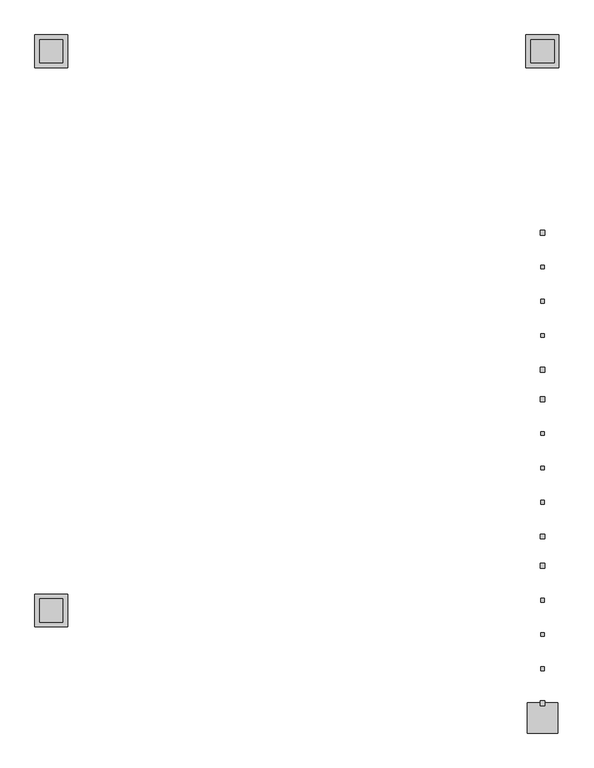
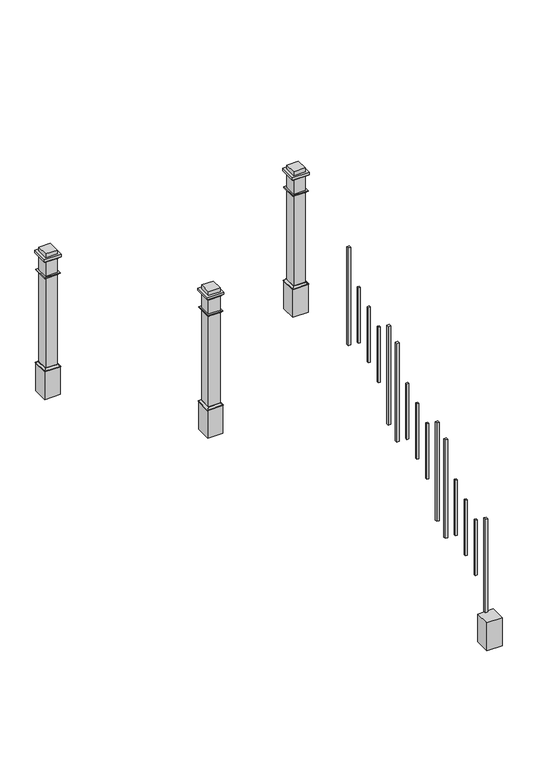
"""IFC4 building model written with IfcOpenShell, lengths in millimetres: railing geometry."""

import ifcopenshell
import ifcopenshell.guid

model = None  # the IFC model being written
_history = None  # IfcOwnerHistory: only IFC2X3 demands one
_inside = {}  # id of a spatial element -> (the spatial element, [elements in it])
_under = {}  # id of a project, library or spatial element -> (it, [spatial elements below it])
_declared = {}  # id of a project -> (the project, [libraries it declares])
_typed = {}  # id of a type object -> (the type object, [elements of that type])
_made_of = {}  # id of a material, layer set ... -> (it, [elements and type objects made of it])


def new_model(schema):
    """Start an empty IFC model of exactly this schema.

    Asked for "IFC4X3", IfcOpenShell would pick the latest addendum, in which some entities
    have other attributes; the version numbers below select the first issue.
    IFC2X3 requires an IfcOwnerHistory on every rooted entity: one is made here for all.
    """
    global model, _history
    if schema == "IFC4X3":
        model = ifcopenshell.file(schema_version=(4, 3, 0, 0))
    else:
        model = ifcopenshell.file(schema=schema)
    _inside.clear()
    _under.clear()
    _declared.clear()
    _typed.clear()
    _made_of.clear()
    _history = None
    if model.schema == "IFC2X3":
        org = make("IfcOrganization", Name="unknown")
        user = make(
            "IfcPersonAndOrganization",
            ThePerson=make("IfcPerson", FamilyName="unknown"),
            TheOrganization=org,
        )
        app = make(
            "IfcApplication",
            ApplicationDeveloper=org,
            Version="unknown",
            ApplicationFullName="unknown",
            ApplicationIdentifier="unknown",
        )
        _history = make(
            "IfcOwnerHistory",
            OwningUser=user,
            OwningApplication=app,
            ChangeAction="ADDED",
            CreationDate=0,
        )
    return model


def make(cls, **values):
    """One entity of the class cls with the attributes given. An attribute that is None is left unset."""
    return model.create_entity(
        cls, **{name: value for name, value in values.items() if value is not None}
    )


def rooted(cls, **values):
    """An entity with a GlobalId (a new one), such as an element, a storey or a relation."""
    return make(cls, GlobalId=ifcopenshell.guid.new(), OwnerHistory=_history, **values)


def si_unit(unit_type, name, prefix=None):
    """IfcSIUnit, for example si_unit("LENGTHUNIT", "METRE", prefix="MILLI")."""
    return make("IfcSIUnit", UnitType=unit_type, Prefix=prefix, Name=name)


def assignment(units):
    """IfcUnitAssignment: the units of a project."""
    return None if units is None else make("IfcUnitAssignment", Units=units)


def point(xyz):
    """IfcCartesianPoint."""
    return None if xyz is None else make("IfcCartesianPoint", Coordinates=xyz)


def direction(xyz):
    """IfcDirection."""
    return None if xyz is None else make("IfcDirection", DirectionRatios=xyz)


def frame(location, z_axis=None, x_axis=None):
    """IfcAxis2Placement3D, a coordinate frame: its origin and axes. An axis left out is left unset."""
    return make(
        "IfcAxis2Placement3D",
        Location=point(location),
        Axis=direction(z_axis),
        RefDirection=direction(x_axis),
    )


def origin():
    """The frame at (0, 0, 0) with its axes left unset."""
    return frame((0.0, 0.0, 0.0))


def place(relative_to, where):
    """IfcLocalPlacement: puts the frame where relative to a parent placement (None: the world)."""
    return make(
        "IfcLocalPlacement", PlacementRelTo=relative_to, RelativePlacement=where
    )


def context(
    kind, dimensions, precision=None, world=None, true_north=None, identifier=None
):
    """IfcGeometricRepresentationContext, for example the 3D "Model" context."""
    return make(
        "IfcGeometricRepresentationContext",
        ContextIdentifier=identifier,
        ContextType=kind,
        CoordinateSpaceDimension=dimensions,
        Precision=precision,
        WorldCoordinateSystem=world,
        TrueNorth=true_north,
    )


def project(units=None, contexts=None):
    """IfcProject with its units and contexts."""
    return rooted(
        "IfcProject",
        Name="project",
        RepresentationContexts=contexts,
        UnitsInContext=assignment(units),
    )


def spatial(cls, under=None, at=None, **own):
    """A site, building, storey or space (cls), placed at a placement, below another one or the project."""
    s = rooted(cls, ObjectPlacement=at, **own)
    if under is not None:
        _under.setdefault(under.id(), (under, []))[1].append(s)
    return s


def polyline(points):
    """IfcPolyline through the points."""
    return make("IfcPolyline", Points=[point(p) for p in points])


def ellipse_curve(where, semi_axis1, semi_axis2):
    """IfcEllipse in the frame where."""
    return make(
        "IfcEllipse", Position=where, SemiAxis1=semi_axis1, SemiAxis2=semi_axis2
    )


def outline(outer, holes=None, kind="AREA"):
    """IfcArbitraryClosedProfileDef: a profile drawn as a closed curve; with holes, ...WithVoids."""
    if holes is None:
        return make("IfcArbitraryClosedProfileDef", ProfileType=kind, OuterCurve=outer)
    return make(
        "IfcArbitraryProfileDefWithVoids",
        ProfileType=kind,
        OuterCurve=outer,
        InnerCurves=holes,
    )


def extrude(swept, where, along, depth):
    """IfcExtrudedAreaSolid: the profile swept, set in the frame where, extruded along a direction by depth."""
    return make(
        "IfcExtrudedAreaSolid",
        SweptArea=swept,
        Position=where,
        ExtrudedDirection=direction(along),
        Depth=depth,
    )


def faces_of(points, faces, orient=None, outer=None):
    """IfcFace entities. A face is a list of loops; a loop is a list of indices into points, from 0.

    orient and outer hold one flag for each loop. By default every Orientation is true, the
    first loop of a face is its IfcFaceOuterBound and the others are IfcFaceBound.
    """
    made = []
    for i, loops in enumerate(faces):
        bounds = []
        for j, loop in enumerate(loops):
            is_outer = j == 0 if outer is None else outer[i][j]
            bounds.append(
                make(
                    "IfcFaceOuterBound" if is_outer else "IfcFaceBound",
                    Bound=make("IfcPolyLoop", Polygon=[points[k] for k in loop]),
                    Orientation=True if orient is None else orient[i][j],
                )
            )
        made.append(make("IfcFace", Bounds=bounds))
    return made


def faceted_brep(points, faces, orient=None, outer=None, voids=None):
    """IfcFacetedBrep: a solid bounded by flat faces; with voids (closed shells), ...WithVoids."""
    shared = [point(p) for p in points]
    hull = make("IfcClosedShell", CfsFaces=faces_of(shared, faces, orient, outer))
    if voids is None:
        return make("IfcFacetedBrep", Outer=hull)
    return make(
        "IfcFacetedBrepWithVoids",
        Outer=hull,
        Voids=[
            make(cls, CfsFaces=faces_of(shared, fs, o, b)) for cls, fs, o, b in voids
        ],
    )


def shape(context_of_items, identifier, shape_type, items):
    """IfcShapeRepresentation: the items that make up one representation, for example the "Body"."""
    return make(
        "IfcShapeRepresentation",
        ContextOfItems=context_of_items,
        RepresentationIdentifier=identifier,
        RepresentationType=shape_type,
        Items=items,
    )


def source(mapping_origin, context_of_items, identifier, shape_type, items):
    """IfcRepresentationMap: a shape defined once, which mapped items show again and again."""
    return make(
        "IfcRepresentationMap",
        MappingOrigin=mapping_origin,
        MappedRepresentation=shape(context_of_items, identifier, shape_type, items),
    )


def transform(
    local_origin,
    x_axis=None,
    y_axis=None,
    z_axis=None,
    scale=None,
    scale2=None,
    scale3=None,
    uniform=True,
):
    """IfcCartesianTransformationOperator3D, or its non-uniform kind. x_axis, y_axis, z_axis: its Axis1, 2, 3."""
    if uniform:
        return make(
            "IfcCartesianTransformationOperator3D",
            Axis1=direction(x_axis),
            Axis2=direction(y_axis),
            LocalOrigin=point(local_origin),
            Scale=scale,
            Axis3=direction(z_axis),
        )
    return make(
        "IfcCartesianTransformationOperator3DnonUniform",
        Axis1=direction(x_axis),
        Axis2=direction(y_axis),
        LocalOrigin=point(local_origin),
        Scale=scale,
        Axis3=direction(z_axis),
        Scale2=scale2,
        Scale3=scale3,
    )


def mapped(mapping_source, mapping_target):
    """IfcMappedItem: shows the shape of a source again, moved by a transform."""
    return make(
        "IfcMappedItem", MappingSource=mapping_source, MappingTarget=mapping_target
    )


def made_of(thing, what):
    """Note that an element or type object is made of a material, layer set ...; save() writes the relation."""
    if what is not None:
        _made_of.setdefault(what.id(), (what, []))[1].append(thing)
    return thing


def element(
    cls,
    number,
    at=None,
    inside=None,
    cuts=None,
    type_object=None,
    material=None,
    context=None,
    identifier="Body",
    shape_type=None,
    held_by="IfcProductDefinitionShape",
    body=None,
    shapes=None,
    **own,
):
    """One element of the class cls, such as IfcWall. Its Tag is "e" and its number.

    at: its placement. inside: the storey or other place that contains it. cuts: it is an
    opening in that element (IfcRelVoidsElement). A single representation is given by context,
    identifier, shape_type and body (its items); several are given by shapes. held_by: the class
    of the entity that holds the representations. save() writes the other relations.
    """
    e = rooted(cls, Tag="e%d" % number, ObjectPlacement=at, **own)
    if body is not None:
        shapes = [shape(context, identifier, shape_type, body)]
    if shapes is not None:
        e.Representation = make(held_by, Representations=shapes)
    if inside is not None:
        _inside.setdefault(inside.id(), (inside, []))[1].append(e)
    if cuts is not None:
        rooted(
            "IfcRelVoidsElement", RelatingBuildingElement=cuts, RelatedOpeningElement=e
        )
    if type_object is not None:
        _typed.setdefault(type_object.id(), (type_object, []))[1].append(e)
    return made_of(e, material)


def aggregate(whole, parts):
    """IfcRelAggregates: a whole, such as a stair, and the parts it consists of."""
    return rooted("IfcRelAggregates", RelatingObject=whole, RelatedObjects=parts)


def save(model, path):
    """Write the relations noted so far, then the file.

    IfcRelAggregates (storeys below a building ...), IfcRelContainedInSpatialStructure (elements
    in a storey), IfcRelDefinesByType, IfcRelAssociatesMaterial and IfcRelDeclares: one each for
    every whole, place, type object, material and project.
    """
    for whole, parts in _under.values():
        aggregate(whole, parts)
    for where, things in _inside.values():
        rooted(
            "IfcRelContainedInSpatialStructure",
            RelatedElements=things,
            RelatingStructure=where,
        )
    for kind, things in _typed.values():
        rooted("IfcRelDefinesByType", RelatedObjects=things, RelatingType=kind)
    for what, things in _made_of.values():
        rooted("IfcRelAssociatesMaterial", RelatedObjects=things, RelatingMaterial=what)
    for by, libraries in _declared.values():
        rooted("IfcRelDeclares", RelatingContext=by, RelatedDefinitions=libraries)
    model.write(path)


def plane_surface(at):
    """IfcPlane: the flat surface through the origin of the frame at, square to its z axis."""
    return make("IfcPlane", Position=at)


def revolved_surface(curve, axis_point, axis_direction):
    """IfcSurfaceOfRevolution: the curve turned about the line through axis_point along axis_direction."""
    return make(
        "IfcSurfaceOfRevolution",
        SweptCurve=make("IfcArbitraryOpenProfileDef", ProfileType="CURVE", Curve=curve),
        AxisPosition=make("IfcAxis1Placement", Location=point(axis_point), Axis=direction(axis_direction)),
    )


def advanced_brep(points, edges, surfaces, faces):
    """IfcAdvancedBrep: a solid bounded by faces that lie on surfaces and meet in shared edges.

    An edge is (start, end): straight between two places in points (the first is 0);
    or (start, end, curve); or (start, end, curve, False) where it runs against its curve.
    A face is (place in surfaces, loops), or (place, loops, False) where it looks against
    its surface's normal. A loop lists edges by number (the first is 1), with a minus sign
    where the edge is run from its end to its start. The first loop is the outer one.
    """
    corners = [point(p) for p in points]
    vertices = [make("IfcVertexPoint", VertexGeometry=c) for c in corners]
    made = []
    for start, end, *more in edges:
        made.append(
            make(
                "IfcEdgeCurve",
                EdgeStart=vertices[start],
                EdgeEnd=vertices[end],
                EdgeGeometry=more[0] if more else make("IfcPolyline", Points=[corners[start], corners[end]]),
                SameSense=more[1] if len(more) > 1 else True,
            )
        )
    hull = []
    for where, loops, *sense in faces:
        bounds = []
        for j, loop in enumerate(loops):
            ring = [make("IfcOrientedEdge", EdgeElement=made[abs(k) - 1], Orientation=k > 0) for k in loop]
            bounds.append(
                make(
                    "IfcFaceOuterBound" if j == 0 else "IfcFaceBound",
                    Bound=make("IfcEdgeLoop", EdgeList=ring),
                    Orientation=True,
                )
            )
        hull.append(make("IfcAdvancedFace", Bounds=bounds, FaceSurface=surfaces[where], SameSense=sense[0] if sense else True))
    return make("IfcAdvancedBrep", Outer=make("IfcClosedShell", CfsFaces=hull))


def railing_a93c2c6f(model_context):
    return source(origin(), model_context, "Body", "SolidModel", [
        extrude(outline(polyline([(-18256.4384928, 383.6340384), (-18281.8384928, 383.6340384), (-18281.8384928, 409.0340384), (-18256.4384928, 409.0340384), (-18256.4384928, 383.6340384)])), frame((0.0, 0.0, 1692.8814161), z_axis=(0.0, 0.0, 1.0), x_axis=(1.0, 0.0, 0.0)), (0.0, 0.0, 1.0), 1067.2519172),
        extrude(outline(polyline([(-18259.6134928, 208.0898059), (-18278.6634928, 208.0898059), (-18278.6634928, 227.1398059), (-18259.6134928, 227.1398059), (-18259.6134928, 208.0898059)])), frame((0.0, 0.0, 1825.7985131), z_axis=(0.0, 0.0, 1.0), x_axis=(1.0, 0.0, 0.0)), (0.0, 0.0, 1.0), 605.2992699),
        extrude(outline(polyline([(-18259.6134928, 29.3705733), (-18278.6634928, 29.3705733), (-18278.6634928, 48.4205733), (-18259.6134928, 48.4205733), (-18259.6134928, 29.3705733)])), frame((0.0, 0.0, 1717.4838267), z_axis=(0.0, 0.0, 1.0), x_axis=(1.0, 0.0, 0.0)), (0.0, 0.0, 1.0), 605.2992699),
        extrude(outline(polyline([(-18259.6134928, -149.3486592), (-18278.6634928, -149.3486592), (-18278.6634928, -130.2986592), (-18259.6134928, -130.2986592), (-18259.6134928, -149.3486592)])), frame((0.0, 0.0, 1609.1691403), z_axis=(0.0, 0.0, 1.0), x_axis=(1.0, 0.0, 0.0)), (0.0, 0.0, 1.0), 605.2992699),
        extrude(outline(polyline([(-18256.4384928, -331.2428917), (-18281.8384928, -331.2428917), (-18281.8384928, -305.8428917), (-18256.4384928, -305.8428917), (-18256.4384928, -331.2428917)])), frame((0.0, 0.0, 1259.6226706), z_axis=(0.0, 0.0, 1.0), x_axis=(1.0, 0.0, 0.0)), (0.0, 0.0, 1.0), 1075.1310532),
        extrude(outline(polyline([(-18256.4384928, -484.4308054), (-18281.8384928, -484.4308054), (-18281.8384928, -459.0308054), (-18256.4384928, -459.0308054), (-18256.4384928, -484.4308054)])), frame((0.0, 0.0, 1166.7815108), z_axis=(0.0, 0.0, 1.0), x_axis=(1.0, 0.0, 0.0)), (0.0, 0.0, 1.0), 1075.1310532),
        extrude(outline(polyline([(-18259.6134928, -659.9750379), (-18278.6634928, -659.9750379), (-18278.6634928, -640.9250379), (-18259.6134928, -640.9250379), (-18259.6134928, -659.9750379)])), frame((0.0, 0.0, 1299.6986078), z_axis=(0.0, 0.0, 1.0), x_axis=(1.0, 0.0, 0.0)), (0.0, 0.0, 1.0), 605.2992699),
        extrude(outline(polyline([(-18259.6134928, -838.6942704), (-18278.6634928, -838.6942704), (-18278.6634928, -819.6442704), (-18259.6134928, -819.6442704), (-18259.6134928, -838.6942704)])), frame((0.0, 0.0, 1191.3839214), z_axis=(0.0, 0.0, 1.0), x_axis=(1.0, 0.0, 0.0)), (0.0, 0.0, 1.0), 605.2992699),
        extrude(outline(polyline([(-18259.6134928, -1017.413503), (-18278.6634928, -1017.413503), (-18278.6634928, -998.363503), (-18259.6134928, -998.363503), (-18259.6134928, -1017.413503)])), frame((0.0, 0.0, 1083.069235), z_axis=(0.0, 0.0, 1.0), x_axis=(1.0, 0.0, 0.0)), (0.0, 0.0, 1.0), 605.2992699),
        extrude(outline(polyline([(-18256.4384928, -1199.3077355), (-18281.8384928, -1199.3077355), (-18281.8384928, -1173.9077355), (-18256.4384928, -1173.9077355), (-18256.4384928, -1199.3077355)])), frame((0.0, 0.0, 733.5227653), z_axis=(0.0, 0.0, 1.0), x_axis=(1.0, 0.0, 0.0)), (0.0, 0.0, 1.0), 1075.1310532),
        extrude(outline(polyline([(-18256.4384928, -1352.4956491), (-18281.8384928, -1352.4956491), (-18281.8384928, -1327.0956491), (-18256.4384928, -1327.0956491), (-18256.4384928, -1352.4956491)])), frame((0.0, 0.0, 640.6816055), z_axis=(0.0, 0.0, 1.0), x_axis=(1.0, 0.0, 0.0)), (0.0, 0.0, 1.0), 1075.1310532),
        extrude(outline(polyline([(-18259.6134928, -1528.0398816), (-18278.6634928, -1528.0398816), (-18278.6634928, -1508.9898816), (-18259.6134928, -1508.9898816), (-18259.6134928, -1528.0398816)])), frame((0.0, 0.0, 773.5987025), z_axis=(0.0, 0.0, 1.0), x_axis=(1.0, 0.0, 0.0)), (0.0, 0.0, 1.0), 605.2992699),
        extrude(outline(polyline([(-18259.6134928, -1706.7591142), (-18278.6634928, -1706.7591142), (-18278.6634928, -1687.7091142), (-18259.6134928, -1687.7091142), (-18259.6134928, -1706.7591142)])), frame((0.0, 0.0, 665.2840161), z_axis=(0.0, 0.0, 1.0), x_axis=(1.0, 0.0, 0.0)), (0.0, 0.0, 1.0), 605.2992699),
        extrude(outline(polyline([(-18259.6134928, -1885.4783467), (-18278.6634928, -1885.4783467), (-18278.6634928, -1866.4283467), (-18259.6134928, -1866.4283467), (-18259.6134928, -1885.4783467)])), frame((0.0, 0.0, 556.9693297), z_axis=(0.0, 0.0, 1.0), x_axis=(1.0, 0.0, 0.0)), (0.0, 0.0, 1.0), 605.2992699),
        extrude(outline(polyline([(-18256.4384928, -2067.3725792), (-18281.8384928, -2067.3725792), (-18281.8384928, -2041.9725792), (-18256.4384928, -2041.9725792), (-18256.4384928, -2067.3725792)])), frame((0.0, 0.0, 207.42286), z_axis=(0.0, 0.0, 1.0), x_axis=(1.0, 0.0, 0.0)), (0.0, 0.0, 1.0), 1075.1310532),
        extrude(outline(polyline([(-20751.3587559, 1261.617839), (-20910.1087559, 1261.617839), (-20910.1087559, 1420.367839), (-20751.3587559, 1420.367839), (-20751.3587559, 1261.617839)])), frame((0.0, 0.0, 1492.5303208), z_axis=(0.0, 0.0, 1.0), x_axis=(1.0, 0.0, 0.0)), (0.0, 0.0, 1.0), 304.8),
        extrude(outline(polyline([(-20770.4087559, 1280.667839), (-20891.0587559, 1280.667839), (-20891.0587559, 1401.317839), (-20770.4087559, 1401.317839), (-20770.4087559, 1280.667839)])), frame((0.0, 0.0, 1797.3303208), z_axis=(0.0, 0.0, 1.0), x_axis=(1.0, 0.0, 0.0)), (0.0, 0.0, 1.0), 1267.6030125),
        extrude(outline(polyline([(-20745.0087559, 1426.717839), (-20745.0087559, 1255.267839), (-20916.4587559, 1255.267839), (-20916.4587559, 1426.717839), (-20745.0087559, 1426.717839)]), holes=[polyline([(-20891.0587559, 1401.317839), (-20891.0587559, 1280.667839), (-20770.4087559, 1280.667839), (-20770.4087559, 1401.317839), (-20891.0587559, 1401.317839)])]), frame((0.0, 0.0, 2998.2583333), z_axis=(0.0, 0.0, 1.0), x_axis=(1.0, 0.0, 0.0)), (0.0, 0.0, 1.0), 25.4),
        advanced_brep(
        [(-20770.4087559, 1401.317839, 1797.3303208), (-20770.4087559, 1401.317839, 1819.5553208), (-20891.0587559, 1401.317839, 1819.5553208), (-20891.0587559, 1401.317839, 1797.3303208), (-20748.1837559, 1423.542839, 1803.6803208), (-20748.1837559, 1423.542839, 1797.3303208), (-20913.2837559, 1423.542839, 1797.3303208), (-20913.2837559, 1423.542839, 1803.6803208), (-20764.0587559, 1407.667839, 1819.5553208), (-20897.4087559, 1407.667839, 1819.5553208), (-20891.0587559, 1280.667839, 1819.5553208), (-20891.0587559, 1280.667839, 1797.3303208), (-20913.2837559, 1258.442839, 1797.3303208), (-20913.2837559, 1258.442839, 1803.6803208), (-20897.4087559, 1274.317839, 1819.5553208), (-20770.4087559, 1280.667839, 1819.5553208), (-20770.4087559, 1280.667839, 1797.3303208), (-20748.1837559, 1258.442839, 1797.3303208), (-20748.1837559, 1258.442839, 1803.6803208), (-20764.0587559, 1274.317839, 1819.5553208)],
        [
            (0, 1),
            (1, 2),
            (2, 3),
            (3, 0),
            (4, 5),
            (5, 6),
            (6, 7),
            (7, 4),
            (8, 4, ellipse_curve(frame((-20748.1837559, 1423.542839, 1819.5553208), z_axis=(0.7071067811865475, -0.7071067811865475, 0.0), x_axis=(-0.7071067811865476, -0.7071067811865474, 0.0)), 22.4506403, 15.875)),
            (7, 9, ellipse_curve(frame((-20913.2837559, 1423.542839, 1819.5553208), z_axis=(-0.7071067811865475, -0.7071067811865475, 0.0), x_axis=(-0.7071067811865476, 0.7071067811865474, 0.0)), 22.4506403, 15.875)),
            (9, 8),
            (2, 10),
            (10, 11),
            (11, 3),
            (6, 12),
            (12, 13),
            (13, 7),
            (13, 14, ellipse_curve(frame((-20913.2837559, 1258.442839, 1819.5553208), z_axis=(0.7071067811865475, -0.7071067811865475, 0.0), x_axis=(-0.7071067811865474, -0.7071067811865476, 0.0)), 22.4506403, 15.875)),
            (14, 9),
            (10, 15),
            (15, 16),
            (16, 11),
            (12, 17),
            (17, 18),
            (18, 13),
            (18, 19, ellipse_curve(frame((-20748.1837559, 1258.442839, 1819.5553208), z_axis=(0.7071067811865475, 0.7071067811865475, 0.0), x_axis=(0.7071067811865476, -0.7071067811865474, 0.0)), 22.4506403, 15.875)),
            (19, 14),
            (15, 1),
            (0, 16),
            (5, 17),
            (4, 18),
            (8, 19),
        ],
        [
            plane_surface(frame((-20770.4087559, 1401.317839, 1819.5553208), z_axis=(0.0, -1.0, 0.0), x_axis=(-1.0, 0.0, 0.0))),
            plane_surface(frame((-20748.1837559, 1423.542839, 1797.3303208), z_axis=(0.0, 1.0, 0.0), x_axis=(-1.0, 0.0, 0.0))),
            revolved_surface(polyline([(-20929.15875589811, 1407.667839, 1819.5553208), (-20732.308755901893, 1407.667839, 1819.5553208)]), (-20770.4087559, 1423.542839, 1819.5553208), (-1.0, 0.0, 0.0)),
            plane_surface(frame((-20891.0587559, 1401.317839, 1819.5553208), z_axis=(1.0, 0.0, 0.0), x_axis=(0.0, -1.0, 0.0))),
            plane_surface(frame((-20913.2837559, 1423.542839, 1797.3303208), z_axis=(-1.0, 0.0, 0.0), x_axis=(0.0, -1.0, 0.0))),
            revolved_surface(polyline([(-20897.4087559, 1242.56783900189, 1819.5553208), (-20897.4087559, 1439.41783899811, 1819.5553208)]), (-20913.2837559, 1401.317839, 1819.5553208), (0.0, -1.0, 0.0)),
            plane_surface(frame((-20891.0587559, 1280.667839, 1819.5553208), z_axis=(0.0, 1.0, 0.0), x_axis=(1.0, 0.0, 0.0))),
            plane_surface(frame((-20913.2837559, 1258.442839, 1797.3303208), z_axis=(0.0, -1.0, 0.0), x_axis=(1.0, 0.0, 0.0))),
            revolved_surface(polyline([(-20732.308755901893, 1274.317839, 1819.5553208), (-20929.15875589811, 1274.317839, 1819.5553208)]), (-20891.0587559, 1258.442839, 1819.5553208), (1.0, 0.0, 0.0)),
            plane_surface(frame((-20770.4087559, 1280.667839, 1819.5553208), z_axis=(-1.0, 0.0, 0.0), x_axis=(0.0, 1.0, 0.0))),
            plane_surface(frame((-20770.4087559, 1280.667839, 1797.3303208), z_axis=(0.0, 0.0, -1.0), x_axis=(0.0, 1.0, 0.0))),
            plane_surface(frame((-20748.1837559, 1258.442839, 1797.3303208), z_axis=(1.0, 0.0, 0.0), x_axis=(0.0, 1.0, 0.0))),
            revolved_surface(polyline([(-20764.0587559, 1439.41783899811, 1819.5553208), (-20764.0587559, 1242.56783900189, 1819.5553208)]), (-20748.1837559, 1280.667839, 1819.5553208), (0.0, 1.0, 0.0)),
            plane_surface(frame((-20764.0587559, 1274.317839, 1819.5553208), z_axis=(0.0, 0.0, 1.0), x_axis=(0.0, 1.0, 0.0))),
        ],
        [
            (0, [[1, 2, 3, 4]]),
            (1, [[5, 6, 7, 8]]),
            (2, [[9, -8, 10, 11]]),
            (3, [[-3, 12, 13, 14]]),
            (4, [[-7, 15, 16, 17]]),
            (5, [[-10, -17, 18, 19]]),
            (6, [[-13, 20, 21, 22]]),
            (7, [[-16, 23, 24, 25]]),
            (8, [[-18, -25, 26, 27]]),
            (9, [[-21, 28, -1, 29]]),
            (10, [[30, -23, -15, -6], [-14, -22, -29, -4]]),
            (11, [[-24, -30, -5, 31]]),
            (12, [[-26, -31, -9, 32]]),
            (13, [[-19, -27, -32, -11], [-28, -20, -12, -2]]),
        ],
    ),
        advanced_brep(
        [(-20770.4087559, 1401.317839, 2801.4083333), (-20770.4087559, 1401.317839, 2820.4583333), (-20891.0587559, 1401.317839, 2820.4583333), (-20891.0587559, 1401.317839, 2801.4083333), (-20751.3587559, 1420.367839, 2814.1083333), (-20764.0587559, 1407.667839, 2801.4083333), (-20897.4087559, 1407.667839, 2801.4083333), (-20910.1087559, 1420.367839, 2814.1083333), (-20751.3587559, 1420.367839, 2820.4583333), (-20910.1087559, 1420.367839, 2820.4583333), (-20891.0587559, 1280.667839, 2820.4583333), (-20891.0587559, 1280.667839, 2801.4083333), (-20897.4087559, 1274.317839, 2801.4083333), (-20910.1087559, 1261.617839, 2814.1083333), (-20910.1087559, 1261.617839, 2820.4583333), (-20770.4087559, 1280.667839, 2820.4583333), (-20770.4087559, 1280.667839, 2801.4083333), (-20764.0587559, 1274.317839, 2801.4083333), (-20751.3587559, 1261.617839, 2814.1083333), (-20751.3587559, 1261.617839, 2820.4583333)],
        [
            (0, 1),
            (1, 2),
            (2, 3),
            (3, 0),
            (4, 5, ellipse_curve(frame((-20751.3587559, 1420.367839, 2801.4083333), z_axis=(0.7071067811865475, -0.7071067811865475, 0.0), x_axis=(-0.7071067811865476, -0.7071067811865474, 0.0)), 17.9605122, 12.7)),
            (5, 6),
            (6, 7, ellipse_curve(frame((-20910.1087559, 1420.367839, 2801.4083333), z_axis=(-0.7071067811865475, -0.7071067811865475, 0.0), x_axis=(-0.7071067811865476, 0.7071067811865474, 0.0)), 17.9605122, 12.7)),
            (7, 4),
            (8, 4),
            (7, 9),
            (9, 8),
            (2, 10),
            (10, 11),
            (11, 3),
            (6, 12),
            (12, 13, ellipse_curve(frame((-20910.1087559, 1261.617839, 2801.4083333), z_axis=(0.7071067811865475, -0.7071067811865475, 0.0), x_axis=(-0.7071067811865474, -0.7071067811865476, 0.0)), 17.9605122, 12.7)),
            (13, 7),
            (13, 14),
            (14, 9),
            (10, 15),
            (15, 16),
            (16, 11),
            (12, 17),
            (17, 18, ellipse_curve(frame((-20751.3587559, 1261.617839, 2801.4083333), z_axis=(0.7071067811865475, 0.7071067811865475, 0.0), x_axis=(0.7071067811865476, -0.7071067811865474, 0.0)), 17.9605122, 12.7)),
            (18, 13),
            (18, 19),
            (19, 14),
            (19, 8),
            (1, 15),
            (0, 16),
            (5, 17),
            (4, 18),
        ],
        [
            plane_surface(frame((-20770.4087559, 1401.317839, 2820.4583333), z_axis=(0.0, -1.0, 0.0), x_axis=(-1.0, 0.0, 0.0))),
            revolved_surface(polyline([(-20922.808755870203, 1407.667839, 2801.4083333), (-20738.6587559298, 1407.667839, 2801.4083333)]), (-20770.4087559, 1420.367839, 2801.4083333), (-1.0, 0.0, 0.0)),
            plane_surface(frame((-20751.3587559, 1420.367839, 2814.1083333), z_axis=(0.0, 1.0, 0.0), x_axis=(-1.0, 0.0, 0.0))),
            plane_surface(frame((-20891.0587559, 1401.317839, 2820.4583333), z_axis=(1.0, 0.0, 0.0), x_axis=(0.0, -1.0, 0.0))),
            revolved_surface(polyline([(-20897.4087559, 1248.9178390297964, 2801.4083333), (-20897.4087559, 1433.0678389702036, 2801.4083333)]), (-20910.1087559, 1401.317839, 2801.4083333), (0.0, -1.0, 0.0)),
            plane_surface(frame((-20910.1087559, 1420.367839, 2814.1083333), z_axis=(-1.0, 0.0, 0.0), x_axis=(0.0, -1.0, 0.0))),
            plane_surface(frame((-20891.0587559, 1280.667839, 2820.4583333), z_axis=(0.0, 1.0, 0.0), x_axis=(1.0, 0.0, 0.0))),
            revolved_surface(polyline([(-20738.6587559298, 1274.317839, 2801.4083333), (-20922.808755870203, 1274.317839, 2801.4083333)]), (-20891.0587559, 1261.617839, 2801.4083333), (1.0, 0.0, 0.0)),
            plane_surface(frame((-20910.1087559, 1261.617839, 2814.1083333), z_axis=(0.0, -1.0, 0.0), x_axis=(1.0, 0.0, 0.0))),
            plane_surface(frame((-20751.3587559, 1261.617839, 2820.4583333), z_axis=(0.0, 0.0, 1.0), x_axis=(0.0, 1.0, 0.0))),
            plane_surface(frame((-20770.4087559, 1280.667839, 2820.4583333), z_axis=(-1.0, 0.0, 0.0), x_axis=(0.0, 1.0, 0.0))),
            plane_surface(frame((-20770.4087559, 1280.667839, 2801.4083333), z_axis=(0.0, 0.0, -1.0), x_axis=(0.0, 1.0, 0.0))),
            revolved_surface(polyline([(-20764.0587559, 1433.0678389702036, 2801.4083333), (-20764.0587559, 1248.9178390297964, 2801.4083333)]), (-20751.3587559, 1280.667839, 2801.4083333), (0.0, 1.0, 0.0)),
            plane_surface(frame((-20751.3587559, 1261.617839, 2814.1083333), z_axis=(1.0, 0.0, 0.0), x_axis=(0.0, 1.0, 0.0))),
        ],
        [
            (0, [[1, 2, 3, 4]]),
            (1, [[5, 6, 7, 8]]),
            (2, [[9, -8, 10, 11]]),
            (3, [[-3, 12, 13, 14]]),
            (4, [[-7, 15, 16, 17]]),
            (5, [[-10, -17, 18, 19]]),
            (6, [[-13, 20, 21, 22]]),
            (7, [[-16, 23, 24, 25]]),
            (8, [[-18, -25, 26, 27]]),
            (9, [[-19, -27, 28, -11], [29, -20, -12, -2]]),
            (10, [[-21, -29, -1, 30]]),
            (11, [[31, -23, -15, -6], [-14, -22, -30, -4]]),
            (12, [[-24, -31, -5, 32]]),
            (13, [[-26, -32, -9, -28]]),
        ],
    ),
        faceted_brep([(-20770.4087559, 1401.317839, 2979.2083333), (-20770.4087559, 1401.317839, 2998.2583333), (-20891.0587559, 1401.317839, 2998.2583333), (-20891.0587559, 1401.317839, 2979.2083333), (-20764.0587559, 1407.667839, 2991.9083333), (-20764.0587559, 1407.667839, 2979.2083333), (-20897.4087559, 1407.667839, 2979.2083333), (-20897.4087559, 1407.667839, 2991.9083333), (-20751.3587559, 1420.367839, 2998.2583333), (-20751.3587559, 1420.367839, 2991.9083333), (-20910.1087559, 1420.367839, 2991.9083333), (-20910.1087559, 1420.367839, 2998.2583333), (-20891.0587559, 1280.667839, 2998.2583333), (-20891.0587559, 1280.667839, 2979.2083333), (-20897.4087559, 1274.317839, 2979.2083333), (-20897.4087559, 1274.317839, 2991.9083333), (-20910.1087559, 1261.617839, 2991.9083333), (-20910.1087559, 1261.617839, 2998.2583333), (-20770.4087559, 1280.667839, 2998.2583333), (-20770.4087559, 1280.667839, 2979.2083333), (-20764.0587559, 1274.317839, 2979.2083333), (-20764.0587559, 1274.317839, 2991.9083333), (-20751.3587559, 1261.617839, 2991.9083333), (-20751.3587559, 1261.617839, 2998.2583333)], [[[0, 1, 2, 3]], [[4, 5, 6, 7]], [[8, 9, 10, 11]], [[3, 2, 12, 13]], [[7, 6, 14, 15]], [[11, 10, 16, 17]], [[13, 12, 18, 19]], [[15, 14, 20, 21]], [[17, 16, 22, 23]], [[19, 18, 1, 0]], [[5, 20, 14, 6], [3, 13, 19, 0]], [[21, 20, 5, 4]], [[9, 22, 16, 10], [7, 15, 21, 4]], [[23, 22, 9, 8]], [[11, 17, 23, 8], [1, 18, 12, 2]]]),
        extrude(outline(polyline([(-18348.5134928, 1261.617839), (-18348.5134928, 1420.367839), (-18189.7634928, 1420.367839), (-18189.7634928, 1261.617839), (-18348.5134928, 1261.617839)])), frame((0.0, 0.0, 1492.5303208), z_axis=(0.0, 0.0, 1.0), x_axis=(1.0, 0.0, 0.0)), (0.0, 0.0, 1.0), 304.8),
        extrude(outline(polyline([(-18329.4634928, 1280.667839), (-18329.4634928, 1401.317839), (-18208.8134928, 1401.317839), (-18208.8134928, 1280.667839), (-18329.4634928, 1280.667839)])), frame((0.0, 0.0, 1797.3303208), z_axis=(0.0, 0.0, 1.0), x_axis=(1.0, 0.0, 0.0)), (0.0, 0.0, 1.0), 1267.6030125),
        extrude(outline(polyline([(-18183.4134928, 1255.267839), (-18354.8634928, 1255.267839), (-18354.8634928, 1426.717839), (-18183.4134928, 1426.717839), (-18183.4134928, 1255.267839)]), holes=[polyline([(-18208.8134928, 1401.317839), (-18329.4634928, 1401.317839), (-18329.4634928, 1280.667839), (-18208.8134928, 1280.667839), (-18208.8134928, 1401.317839)])]), frame((0.0, 0.0, 2998.2583333), z_axis=(0.0, 0.0, 1.0), x_axis=(1.0, 0.0, 0.0)), (0.0, 0.0, 1.0), 25.4),
        advanced_brep(
        [(-18208.8134928, 1280.667839, 1797.3303208), (-18208.8134928, 1280.667839, 1819.5553208), (-18208.8134928, 1401.317839, 1819.5553208), (-18208.8134928, 1401.317839, 1797.3303208), (-18186.5884928, 1258.442839, 1803.6803208), (-18186.5884928, 1258.442839, 1797.3303208), (-18186.5884928, 1423.542839, 1797.3303208), (-18186.5884928, 1423.542839, 1803.6803208), (-18202.4634928, 1274.317839, 1819.5553208), (-18202.4634928, 1407.667839, 1819.5553208), (-18329.4634928, 1401.317839, 1819.5553208), (-18329.4634928, 1401.317839, 1797.3303208), (-18351.6884928, 1423.542839, 1797.3303208), (-18351.6884928, 1423.542839, 1803.6803208), (-18335.8134928, 1407.667839, 1819.5553208), (-18329.4634928, 1280.667839, 1819.5553208), (-18329.4634928, 1280.667839, 1797.3303208), (-18351.6884928, 1258.442839, 1797.3303208), (-18351.6884928, 1258.442839, 1803.6803208), (-18335.8134928, 1274.317839, 1819.5553208)],
        [
            (0, 1),
            (1, 2),
            (2, 3),
            (3, 0),
            (4, 5),
            (5, 6),
            (6, 7),
            (7, 4),
            (8, 4, ellipse_curve(frame((-18186.5884928, 1258.442839, 1819.5553208), z_axis=(-0.7071067811865475, -0.7071067811865475, 0.0), x_axis=(-0.7071067811865474, 0.7071067811865476, 0.0)), 22.4506403, 15.875)),
            (7, 9, ellipse_curve(frame((-18186.5884928, 1423.542839, 1819.5553208), z_axis=(-0.7071067811865475, 0.7071067811865475, 0.0), x_axis=(0.7071067811865474, 0.7071067811865476, 0.0)), 22.4506403, 15.875)),
            (9, 8),
            (2, 10),
            (10, 11),
            (11, 3),
            (6, 12),
            (12, 13),
            (13, 7),
            (13, 14, ellipse_curve(frame((-18351.6884928, 1423.542839, 1819.5553208), z_axis=(-0.7071067811865475, -0.7071067811865475, 0.0), x_axis=(-0.7071067811865476, 0.7071067811865474, 0.0)), 22.4506403, 15.875)),
            (14, 9),
            (10, 15),
            (15, 16),
            (16, 11),
            (12, 17),
            (17, 18),
            (18, 13),
            (18, 19, ellipse_curve(frame((-18351.6884928, 1258.442839, 1819.5553208), z_axis=(0.7071067811865475, -0.7071067811865475, 0.0), x_axis=(-0.7071067811865474, -0.7071067811865476, 0.0)), 22.4506403, 15.875)),
            (19, 14),
            (15, 1),
            (0, 16),
            (5, 17),
            (4, 18),
            (8, 19),
        ],
        [
            plane_surface(frame((-18208.8134928, 1280.667839, 1819.5553208), z_axis=(-1.0, 0.0, 0.0), x_axis=(0.0, 1.0, 0.0))),
            plane_surface(frame((-18186.5884928, 1258.442839, 1797.3303208), z_axis=(1.0, 0.0, 0.0), x_axis=(0.0, 1.0, 0.0))),
            revolved_surface(polyline([(-18202.4634928, 1439.41783899811, 1819.5553208), (-18202.4634928, 1242.56783900189, 1819.5553208)]), (-18186.5884928, 1280.667839, 1819.5553208), (0.0, 1.0, 0.0)),
            plane_surface(frame((-18208.8134928, 1401.317839, 1819.5553208), z_axis=(0.0, -1.0, 0.0), x_axis=(-1.0, 0.0, 0.0))),
            plane_surface(frame((-18186.5884928, 1423.542839, 1797.3303208), z_axis=(0.0, 1.0, 0.0), x_axis=(-1.0, 0.0, 0.0))),
            revolved_surface(polyline([(-18367.56349279811, 1407.667839, 1819.5553208), (-18170.713492801893, 1407.667839, 1819.5553208)]), (-18208.8134928, 1423.542839, 1819.5553208), (-1.0, 0.0, 0.0)),
            plane_surface(frame((-18329.4634928, 1401.317839, 1819.5553208), z_axis=(1.0, 0.0, 0.0), x_axis=(0.0, -1.0, 0.0))),
            plane_surface(frame((-18351.6884928, 1423.542839, 1797.3303208), z_axis=(-1.0, 0.0, 0.0), x_axis=(0.0, -1.0, 0.0))),
            revolved_surface(polyline([(-18335.8134928, 1242.56783900189, 1819.5553208), (-18335.8134928, 1439.41783899811, 1819.5553208)]), (-18351.6884928, 1401.317839, 1819.5553208), (0.0, -1.0, 0.0)),
            plane_surface(frame((-18329.4634928, 1280.667839, 1819.5553208), z_axis=(0.0, 1.0, 0.0), x_axis=(1.0, 0.0, 0.0))),
            plane_surface(frame((-18329.4634928, 1280.667839, 1797.3303208), z_axis=(0.0, 0.0, -1.0), x_axis=(1.0, 0.0, 0.0))),
            plane_surface(frame((-18351.6884928, 1258.442839, 1797.3303208), z_axis=(0.0, -1.0, 0.0), x_axis=(1.0, 0.0, 0.0))),
            revolved_surface(polyline([(-18170.713492801893, 1274.317839, 1819.5553208), (-18367.56349279811, 1274.317839, 1819.5553208)]), (-18329.4634928, 1258.442839, 1819.5553208), (1.0, 0.0, 0.0)),
            plane_surface(frame((-18335.8134928, 1274.317839, 1819.5553208), z_axis=(0.0, 0.0, 1.0), x_axis=(1.0, 0.0, 0.0))),
        ],
        [
            (0, [[1, 2, 3, 4]]),
            (1, [[5, 6, 7, 8]]),
            (2, [[9, -8, 10, 11]]),
            (3, [[-3, 12, 13, 14]]),
            (4, [[-7, 15, 16, 17]]),
            (5, [[-10, -17, 18, 19]]),
            (6, [[-13, 20, 21, 22]]),
            (7, [[-16, 23, 24, 25]]),
            (8, [[-18, -25, 26, 27]]),
            (9, [[-21, 28, -1, 29]]),
            (10, [[30, -23, -15, -6], [-14, -22, -29, -4]]),
            (11, [[-24, -30, -5, 31]]),
            (12, [[-26, -31, -9, 32]]),
            (13, [[-19, -27, -32, -11], [-28, -20, -12, -2]]),
        ],
    ),
        advanced_brep(
        [(-18208.8134928, 1280.667839, 2801.4083333), (-18208.8134928, 1280.667839, 2820.4583333), (-18208.8134928, 1401.317839, 2820.4583333), (-18208.8134928, 1401.317839, 2801.4083333), (-18189.7634928, 1261.617839, 2814.1083333), (-18202.4634928, 1274.317839, 2801.4083333), (-18202.4634928, 1407.667839, 2801.4083333), (-18189.7634928, 1420.367839, 2814.1083333), (-18189.7634928, 1261.617839, 2820.4583333), (-18189.7634928, 1420.367839, 2820.4583333), (-18329.4634928, 1401.317839, 2820.4583333), (-18329.4634928, 1401.317839, 2801.4083333), (-18335.8134928, 1407.667839, 2801.4083333), (-18348.5134928, 1420.367839, 2814.1083333), (-18348.5134928, 1420.367839, 2820.4583333), (-18329.4634928, 1280.667839, 2820.4583333), (-18329.4634928, 1280.667839, 2801.4083333), (-18335.8134928, 1274.317839, 2801.4083333), (-18348.5134928, 1261.617839, 2814.1083333), (-18348.5134928, 1261.617839, 2820.4583333)],
        [
            (0, 1),
            (1, 2),
            (2, 3),
            (3, 0),
            (4, 5, ellipse_curve(frame((-18189.7634928, 1261.617839, 2801.4083333), z_axis=(-0.7071067811865475, -0.7071067811865475, 0.0), x_axis=(-0.7071067811865474, 0.7071067811865476, 0.0)), 17.9605122, 12.7)),
            (5, 6),
            (6, 7, ellipse_curve(frame((-18189.7634928, 1420.367839, 2801.4083333), z_axis=(-0.7071067811865475, 0.7071067811865475, 0.0), x_axis=(0.7071067811865474, 0.7071067811865476, 0.0)), 17.9605122, 12.7)),
            (7, 4),
            (8, 4),
            (7, 9),
            (9, 8),
            (2, 10),
            (10, 11),
            (11, 3),
            (6, 12),
            (12, 13, ellipse_curve(frame((-18348.5134928, 1420.367839, 2801.4083333), z_axis=(-0.7071067811865475, -0.7071067811865475, 0.0), x_axis=(-0.7071067811865476, 0.7071067811865474, 0.0)), 17.9605122, 12.7)),
            (13, 7),
            (13, 14),
            (14, 9),
            (10, 15),
            (15, 16),
            (16, 11),
            (12, 17),
            (17, 18, ellipse_curve(frame((-18348.5134928, 1261.617839, 2801.4083333), z_axis=(0.7071067811865475, -0.7071067811865475, 0.0), x_axis=(-0.7071067811865474, -0.7071067811865476, 0.0)), 17.9605122, 12.7)),
            (18, 13),
            (18, 19),
            (19, 14),
            (19, 8),
            (1, 15),
            (0, 16),
            (5, 17),
            (4, 18),
        ],
        [
            plane_surface(frame((-18208.8134928, 1280.667839, 2820.4583333), z_axis=(-1.0, 0.0, 0.0), x_axis=(0.0, 1.0, 0.0))),
            revolved_surface(polyline([(-18202.4634928, 1433.0678389702036, 2801.4083333), (-18202.4634928, 1248.9178390297964, 2801.4083333)]), (-18189.7634928, 1280.667839, 2801.4083333), (0.0, 1.0, 0.0)),
            plane_surface(frame((-18189.7634928, 1261.617839, 2814.1083333), z_axis=(1.0, 0.0, 0.0), x_axis=(0.0, 1.0, 0.0))),
            plane_surface(frame((-18208.8134928, 1401.317839, 2820.4583333), z_axis=(0.0, -1.0, 0.0), x_axis=(-1.0, 0.0, 0.0))),
            revolved_surface(polyline([(-18361.213492770203, 1407.667839, 2801.4083333), (-18177.0634928298, 1407.667839, 2801.4083333)]), (-18208.8134928, 1420.367839, 2801.4083333), (-1.0, 0.0, 0.0)),
            plane_surface(frame((-18189.7634928, 1420.367839, 2814.1083333), z_axis=(0.0, 1.0, 0.0), x_axis=(-1.0, 0.0, 0.0))),
            plane_surface(frame((-18329.4634928, 1401.317839, 2820.4583333), z_axis=(1.0, 0.0, 0.0), x_axis=(0.0, -1.0, 0.0))),
            revolved_surface(polyline([(-18335.8134928, 1248.9178390297964, 2801.4083333), (-18335.8134928, 1433.0678389702036, 2801.4083333)]), (-18348.5134928, 1401.317839, 2801.4083333), (0.0, -1.0, 0.0)),
            plane_surface(frame((-18348.5134928, 1420.367839, 2814.1083333), z_axis=(-1.0, 0.0, 0.0), x_axis=(0.0, -1.0, 0.0))),
            plane_surface(frame((-18348.5134928, 1261.617839, 2820.4583333), z_axis=(0.0, 0.0, 1.0), x_axis=(1.0, 0.0, 0.0))),
            plane_surface(frame((-18329.4634928, 1280.667839, 2820.4583333), z_axis=(0.0, 1.0, 0.0), x_axis=(1.0, 0.0, 0.0))),
            plane_surface(frame((-18329.4634928, 1280.667839, 2801.4083333), z_axis=(0.0, 0.0, -1.0), x_axis=(1.0, 0.0, 0.0))),
            revolved_surface(polyline([(-18177.0634928298, 1274.317839, 2801.4083333), (-18361.213492770203, 1274.317839, 2801.4083333)]), (-18329.4634928, 1261.617839, 2801.4083333), (1.0, 0.0, 0.0)),
            plane_surface(frame((-18348.5134928, 1261.617839, 2814.1083333), z_axis=(0.0, -1.0, 0.0), x_axis=(1.0, 0.0, 0.0))),
        ],
        [
            (0, [[1, 2, 3, 4]]),
            (1, [[5, 6, 7, 8]]),
            (2, [[9, -8, 10, 11]]),
            (3, [[-3, 12, 13, 14]]),
            (4, [[-7, 15, 16, 17]]),
            (5, [[-10, -17, 18, 19]]),
            (6, [[-13, 20, 21, 22]]),
            (7, [[-16, 23, 24, 25]]),
            (8, [[-18, -25, 26, 27]]),
            (9, [[-19, -27, 28, -11], [29, -20, -12, -2]]),
            (10, [[-21, -29, -1, 30]]),
            (11, [[31, -23, -15, -6], [-14, -22, -30, -4]]),
            (12, [[-24, -31, -5, 32]]),
            (13, [[-26, -32, -9, -28]]),
        ],
    ),
        faceted_brep([(-18208.8134928, 1280.667839, 2979.2083333), (-18208.8134928, 1280.667839, 2998.2583333), (-18208.8134928, 1401.317839, 2998.2583333), (-18208.8134928, 1401.317839, 2979.2083333), (-18202.4634928, 1274.317839, 2991.9083333), (-18202.4634928, 1274.317839, 2979.2083333), (-18202.4634928, 1407.667839, 2979.2083333), (-18202.4634928, 1407.667839, 2991.9083333), (-18189.7634928, 1261.617839, 2998.2583333), (-18189.7634928, 1261.617839, 2991.9083333), (-18189.7634928, 1420.367839, 2991.9083333), (-18189.7634928, 1420.367839, 2998.2583333), (-18329.4634928, 1401.317839, 2998.2583333), (-18329.4634928, 1401.317839, 2979.2083333), (-18335.8134928, 1407.667839, 2979.2083333), (-18335.8134928, 1407.667839, 2991.9083333), (-18348.5134928, 1420.367839, 2991.9083333), (-18348.5134928, 1420.367839, 2998.2583333), (-18329.4634928, 1280.667839, 2998.2583333), (-18329.4634928, 1280.667839, 2979.2083333), (-18335.8134928, 1274.317839, 2979.2083333), (-18335.8134928, 1274.317839, 2991.9083333), (-18348.5134928, 1261.617839, 2991.9083333), (-18348.5134928, 1261.617839, 2998.2583333)], [[[0, 1, 2, 3]], [[4, 5, 6, 7]], [[8, 9, 10, 11]], [[3, 2, 12, 13]], [[7, 6, 14, 15]], [[11, 10, 16, 17]], [[13, 12, 18, 19]], [[15, 14, 20, 21]], [[17, 16, 22, 23]], [[19, 18, 1, 0]], [[5, 20, 14, 6], [3, 13, 19, 0]], [[21, 20, 5, 4]], [[9, 22, 16, 10], [7, 15, 21, 4]], [[23, 22, 9, 8]], [[11, 17, 23, 8], [1, 18, 12, 2]]]),
        extrude(outline(polyline([(-20751.3587559, -1493.091536), (-20751.3587559, -1651.841536), (-20910.1087559, -1651.841536), (-20910.1087559, -1493.091536), (-20751.3587559, -1493.091536)])), frame((0.0, 0.0, 2836.4689468), z_axis=(0.0, 0.0, 1.0), x_axis=(1.0, 0.0, 0.0)), (0.0, 0.0, 1.0), 304.8),
        extrude(outline(polyline([(-20770.4087559, -1512.141536), (-20770.4087559, -1632.791536), (-20891.0587559, -1632.791536), (-20891.0587559, -1512.141536), (-20770.4087559, -1512.141536)])), frame((0.0, 0.0, 3141.2689468), z_axis=(0.0, 0.0, 1.0), x_axis=(1.0, 0.0, 0.0)), (0.0, 0.0, 1.0), 1278.3310532),
        extrude(outline(polyline([(-20916.4587559, -1486.741536), (-20745.0087559, -1486.741536), (-20745.0087559, -1658.191536), (-20916.4587559, -1658.191536), (-20916.4587559, -1486.741536)]), holes=[polyline([(-20891.0587559, -1632.791536), (-20770.4087559, -1632.791536), (-20770.4087559, -1512.141536), (-20891.0587559, -1512.141536), (-20891.0587559, -1632.791536)])]), frame((0.0, 0.0, 4352.925), z_axis=(0.0, 0.0, 1.0), x_axis=(1.0, 0.0, 0.0)), (0.0, 0.0, 1.0), 25.4),
        advanced_brep(
        [(-20891.0587559, -1512.141536, 3141.2689468), (-20891.0587559, -1512.141536, 3163.4939468), (-20891.0587559, -1632.791536, 3163.4939468), (-20891.0587559, -1632.791536, 3141.2689468), (-20913.2837559, -1489.916536, 3147.6189468), (-20913.2837559, -1489.916536, 3141.2689468), (-20913.2837559, -1655.016536, 3141.2689468), (-20913.2837559, -1655.016536, 3147.6189468), (-20897.4087559, -1505.791536, 3163.4939468), (-20897.4087559, -1639.141536, 3163.4939468), (-20770.4087559, -1632.791536, 3163.4939468), (-20770.4087559, -1632.791536, 3141.2689468), (-20748.1837559, -1655.016536, 3141.2689468), (-20748.1837559, -1655.016536, 3147.6189468), (-20764.0587559, -1639.141536, 3163.4939468), (-20770.4087559, -1512.141536, 3163.4939468), (-20770.4087559, -1512.141536, 3141.2689468), (-20748.1837559, -1489.916536, 3141.2689468), (-20748.1837559, -1489.916536, 3147.6189468), (-20764.0587559, -1505.791536, 3163.4939468)],
        [
            (0, 1),
            (1, 2),
            (2, 3),
            (3, 0),
            (4, 5),
            (5, 6),
            (6, 7),
            (7, 4),
            (8, 4, ellipse_curve(frame((-20913.2837559, -1489.916536, 3163.4939468), z_axis=(0.7071067811865475, 0.7071067811865475, 0.0), x_axis=(0.7071067811865474, -0.7071067811865476, 0.0)), 22.4506403, 15.875)),
            (7, 9, ellipse_curve(frame((-20913.2837559, -1655.016536, 3163.4939468), z_axis=(0.7071067811865475, -0.7071067811865475, 0.0), x_axis=(-0.7071067811865474, -0.7071067811865476, 0.0)), 22.4506403, 15.875)),
            (9, 8),
            (2, 10),
            (10, 11),
            (11, 3),
            (6, 12),
            (12, 13),
            (13, 7),
            (13, 14, ellipse_curve(frame((-20748.1837559, -1655.016536, 3163.4939468), z_axis=(0.7071067811865475, 0.7071067811865475, 0.0), x_axis=(0.7071067811865476, -0.7071067811865474, 0.0)), 22.4506403, 15.875)),
            (14, 9),
            (10, 15),
            (15, 16),
            (16, 11),
            (12, 17),
            (17, 18),
            (18, 13),
            (18, 19, ellipse_curve(frame((-20748.1837559, -1489.916536, 3163.4939468), z_axis=(-0.7071067811865475, 0.7071067811865475, 0.0), x_axis=(0.7071067811865474, 0.7071067811865476, 0.0)), 22.4506403, 15.875)),
            (19, 14),
            (15, 1),
            (0, 16),
            (5, 17),
            (4, 18),
            (8, 19),
        ],
        [
            plane_surface(frame((-20891.0587559, -1512.141536, 3163.4939468), z_axis=(1.0, 0.0, 0.0), x_axis=(0.0, -1.0, 0.0))),
            plane_surface(frame((-20913.2837559, -1489.916536, 3141.2689468), z_axis=(-1.0, 0.0, 0.0), x_axis=(0.0, -1.0, 0.0))),
            revolved_surface(polyline([(-20897.4087559, -1670.8915359981102, 3163.4939468), (-20897.4087559, -1474.0415360018899, 3163.4939468)]), (-20913.2837559, -1512.141536, 3163.4939468), (0.0, -1.0, 0.0)),
            plane_surface(frame((-20891.0587559, -1632.791536, 3163.4939468), z_axis=(0.0, 1.0, 0.0), x_axis=(1.0, 0.0, 0.0))),
            plane_surface(frame((-20913.2837559, -1655.016536, 3141.2689468), z_axis=(0.0, -1.0, 0.0), x_axis=(1.0, 0.0, 0.0))),
            revolved_surface(polyline([(-20732.308755901893, -1639.141536, 3163.4939468), (-20929.15875589811, -1639.141536, 3163.4939468)]), (-20891.0587559, -1655.016536, 3163.4939468), (1.0, 0.0, 0.0)),
            plane_surface(frame((-20770.4087559, -1632.791536, 3163.4939468), z_axis=(-1.0, 0.0, 0.0), x_axis=(0.0, 1.0, 0.0))),
            plane_surface(frame((-20748.1837559, -1655.016536, 3141.2689468), z_axis=(1.0, 0.0, 0.0), x_axis=(0.0, 1.0, 0.0))),
            revolved_surface(polyline([(-20764.0587559, -1474.0415360018899, 3163.4939468), (-20764.0587559, -1670.8915359981102, 3163.4939468)]), (-20748.1837559, -1632.791536, 3163.4939468), (0.0, 1.0, 0.0)),
            plane_surface(frame((-20770.4087559, -1512.141536, 3163.4939468), z_axis=(0.0, -1.0, 0.0), x_axis=(-1.0, 0.0, 0.0))),
            plane_surface(frame((-20770.4087559, -1512.141536, 3141.2689468), z_axis=(0.0, 0.0, -1.0), x_axis=(-1.0, 0.0, 0.0))),
            plane_surface(frame((-20748.1837559, -1489.916536, 3141.2689468), z_axis=(0.0, 1.0, 0.0), x_axis=(-1.0, 0.0, 0.0))),
            revolved_surface(polyline([(-20929.15875589811, -1505.791536, 3163.4939468), (-20732.308755901893, -1505.791536, 3163.4939468)]), (-20770.4087559, -1489.916536, 3163.4939468), (-1.0, 0.0, 0.0)),
            plane_surface(frame((-20764.0587559, -1505.791536, 3163.4939468), z_axis=(0.0, 0.0, 1.0), x_axis=(-1.0, 0.0, 0.0))),
        ],
        [
            (0, [[1, 2, 3, 4]]),
            (1, [[5, 6, 7, 8]]),
            (2, [[9, -8, 10, 11]]),
            (3, [[-3, 12, 13, 14]]),
            (4, [[-7, 15, 16, 17]]),
            (5, [[-10, -17, 18, 19]]),
            (6, [[-13, 20, 21, 22]]),
            (7, [[-16, 23, 24, 25]]),
            (8, [[-18, -25, 26, 27]]),
            (9, [[-21, 28, -1, 29]]),
            (10, [[30, -23, -15, -6], [-14, -22, -29, -4]]),
            (11, [[-24, -30, -5, 31]]),
            (12, [[-26, -31, -9, 32]]),
            (13, [[-19, -27, -32, -11], [-28, -20, -12, -2]]),
        ],
    ),
        advanced_brep(
        [(-20891.0587559, -1512.141536, 4156.075), (-20891.0587559, -1512.141536, 4175.125), (-20891.0587559, -1632.791536, 4175.125), (-20891.0587559, -1632.791536, 4156.075), (-20910.1087559, -1493.091536, 4168.775), (-20897.4087559, -1505.791536, 4156.075), (-20897.4087559, -1639.141536, 4156.075), (-20910.1087559, -1651.841536, 4168.775), (-20910.1087559, -1493.091536, 4175.125), (-20910.1087559, -1651.841536, 4175.125), (-20770.4087559, -1632.791536, 4175.125), (-20770.4087559, -1632.791536, 4156.075), (-20764.0587559, -1639.141536, 4156.075), (-20751.3587559, -1651.841536, 4168.775), (-20751.3587559, -1651.841536, 4175.125), (-20770.4087559, -1512.141536, 4175.125), (-20770.4087559, -1512.141536, 4156.075), (-20764.0587559, -1505.791536, 4156.075), (-20751.3587559, -1493.091536, 4168.775), (-20751.3587559, -1493.091536, 4175.125)],
        [
            (0, 1),
            (1, 2),
            (2, 3),
            (3, 0),
            (4, 5, ellipse_curve(frame((-20910.1087559, -1493.091536, 4156.075), z_axis=(0.7071067811865475, 0.7071067811865475, 0.0), x_axis=(0.7071067811865474, -0.7071067811865476, 0.0)), 17.9605122, 12.7)),
            (5, 6),
            (6, 7, ellipse_curve(frame((-20910.1087559, -1651.841536, 4156.075), z_axis=(0.7071067811865475, -0.7071067811865475, 0.0), x_axis=(-0.7071067811865474, -0.7071067811865476, 0.0)), 17.9605122, 12.7)),
            (7, 4),
            (8, 4),
            (7, 9),
            (9, 8),
            (2, 10),
            (10, 11),
            (11, 3),
            (6, 12),
            (12, 13, ellipse_curve(frame((-20751.3587559, -1651.841536, 4156.075), z_axis=(0.7071067811865475, 0.7071067811865475, 0.0), x_axis=(0.7071067811865476, -0.7071067811865474, 0.0)), 17.9605122, 12.7)),
            (13, 7),
            (13, 14),
            (14, 9),
            (10, 15),
            (15, 16),
            (16, 11),
            (12, 17),
            (17, 18, ellipse_curve(frame((-20751.3587559, -1493.091536, 4156.075), z_axis=(-0.7071067811865475, 0.7071067811865475, 0.0), x_axis=(0.7071067811865474, 0.7071067811865476, 0.0)), 17.9605122, 12.7)),
            (18, 13),
            (18, 19),
            (19, 14),
            (19, 8),
            (1, 15),
            (0, 16),
            (5, 17),
            (4, 18),
        ],
        [
            plane_surface(frame((-20891.0587559, -1512.141536, 4175.125), z_axis=(1.0, 0.0, 0.0), x_axis=(0.0, -1.0, 0.0))),
            revolved_surface(polyline([(-20897.4087559, -1664.5415359702035, 4156.075), (-20897.4087559, -1480.3915360297963, 4156.075)]), (-20910.1087559, -1512.141536, 4156.075), (0.0, -1.0, 0.0)),
            plane_surface(frame((-20910.1087559, -1493.091536, 4168.775), z_axis=(-1.0, 0.0, 0.0), x_axis=(0.0, -1.0, 0.0))),
            plane_surface(frame((-20891.0587559, -1632.791536, 4175.125), z_axis=(0.0, 1.0, 0.0), x_axis=(1.0, 0.0, 0.0))),
            revolved_surface(polyline([(-20738.6587559298, -1639.1415359999999, 4156.075), (-20922.808755870203, -1639.1415359999999, 4156.075)]), (-20891.0587559, -1651.841536, 4156.075), (1.0, 0.0, 0.0)),
            plane_surface(frame((-20910.1087559, -1651.841536, 4168.775), z_axis=(0.0, -1.0, 0.0), x_axis=(1.0, 0.0, 0.0))),
            plane_surface(frame((-20770.4087559, -1632.791536, 4175.125), z_axis=(-1.0, 0.0, 0.0), x_axis=(0.0, 1.0, 0.0))),
            revolved_surface(polyline([(-20764.0587559, -1480.3915360297963, 4156.075), (-20764.0587559, -1664.5415359702035, 4156.075)]), (-20751.3587559, -1632.791536, 4156.075), (0.0, 1.0, 0.0)),
            plane_surface(frame((-20751.3587559, -1651.841536, 4168.775), z_axis=(1.0, 0.0, 0.0), x_axis=(0.0, 1.0, 0.0))),
            plane_surface(frame((-20751.3587559, -1493.091536, 4175.125), z_axis=(0.0, 0.0, 1.0), x_axis=(-1.0, 0.0, 0.0))),
            plane_surface(frame((-20770.4087559, -1512.141536, 4175.125), z_axis=(0.0, -1.0, 0.0), x_axis=(-1.0, 0.0, 0.0))),
            plane_surface(frame((-20770.4087559, -1512.141536, 4156.075), z_axis=(0.0, 0.0, -1.0), x_axis=(-1.0, 0.0, 0.0))),
            revolved_surface(polyline([(-20922.808755870203, -1505.791536, 4156.075), (-20738.6587559298, -1505.791536, 4156.075)]), (-20770.4087559, -1493.091536, 4156.075), (-1.0, 0.0, 0.0)),
            plane_surface(frame((-20751.3587559, -1493.091536, 4168.775), z_axis=(0.0, 1.0, 0.0), x_axis=(-1.0, 0.0, 0.0))),
        ],
        [
            (0, [[1, 2, 3, 4]]),
            (1, [[5, 6, 7, 8]]),
            (2, [[9, -8, 10, 11]]),
            (3, [[-3, 12, 13, 14]]),
            (4, [[-7, 15, 16, 17]]),
            (5, [[-10, -17, 18, 19]]),
            (6, [[-13, 20, 21, 22]]),
            (7, [[-16, 23, 24, 25]]),
            (8, [[-18, -25, 26, 27]]),
            (9, [[-19, -27, 28, -11], [29, -20, -12, -2]]),
            (10, [[-21, -29, -1, 30]]),
            (11, [[31, -23, -15, -6], [-14, -22, -30, -4]]),
            (12, [[-24, -31, -5, 32]]),
            (13, [[-26, -32, -9, -28]]),
        ],
    ),
        faceted_brep([(-20891.0587559, -1512.141536, 4333.875), (-20891.0587559, -1512.141536, 4352.925), (-20891.0587559, -1632.791536, 4352.925), (-20891.0587559, -1632.791536, 4333.875), (-20897.4087559, -1505.791536, 4346.575), (-20897.4087559, -1505.791536, 4333.875), (-20897.4087559, -1639.141536, 4333.875), (-20897.4087559, -1639.141536, 4346.575), (-20910.1087559, -1493.091536, 4352.925), (-20910.1087559, -1493.091536, 4346.575), (-20910.1087559, -1651.841536, 4346.575), (-20910.1087559, -1651.841536, 4352.925), (-20770.4087559, -1632.791536, 4352.925), (-20770.4087559, -1632.791536, 4333.875), (-20764.0587559, -1639.141536, 4333.875), (-20764.0587559, -1639.141536, 4346.575), (-20751.3587559, -1651.841536, 4346.575), (-20751.3587559, -1651.841536, 4352.925), (-20770.4087559, -1512.141536, 4352.925), (-20770.4087559, -1512.141536, 4333.875), (-20764.0587559, -1505.791536, 4333.875), (-20764.0587559, -1505.791536, 4346.575), (-20751.3587559, -1493.091536, 4346.575), (-20751.3587559, -1493.091536, 4352.925)], [[[0, 1, 2, 3]], [[4, 5, 6, 7]], [[8, 9, 10, 11]], [[3, 2, 12, 13]], [[7, 6, 14, 15]], [[11, 10, 16, 17]], [[13, 12, 18, 19]], [[15, 14, 20, 21]], [[17, 16, 22, 23]], [[19, 18, 1, 0]], [[5, 20, 14, 6], [3, 13, 19, 0]], [[21, 20, 5, 4]], [[9, 22, 16, 10], [7, 15, 21, 4]], [[23, 22, 9, 8]], [[11, 17, 23, 8], [1, 18, 12, 2]]]),
        extrude(outline(polyline([(-18348.5134928, -2210.641536), (-18348.5134928, -2051.891536), (-18189.7634928, -2051.891536), (-18189.7634928, -2210.641536), (-18348.5134928, -2210.641536)])), frame((0.0, 0.0, -42.1977199), z_axis=(0.0, 0.0, 1.0), x_axis=(1.0, 0.0, 0.0)), (0.0, 0.0, 1.0), 304.8),
    ])


if __name__ == "__main__":
    model = new_model("IFC4")
    model_context = context("Model", 3, world=origin())
    ifc_project = project(units=[si_unit("LENGTHUNIT", "METRE", prefix="MILLI")], contexts=[model_context])
    site = spatial("IfcSite", under=ifc_project)
    building = spatial("IfcBuilding", under=site)
    placement = place(None, origin())
    railing_shape = railing_a93c2c6f(model_context)
    element("IfcRailing", 1, at=placement, inside=building, context=model_context, shape_type="MappedRepresentation", body=[
        mapped(railing_shape, transform((0.0, 0.0, 0.0), x_axis=(1.0, 0.0, 0.0), y_axis=(0.0, 1.0, 0.0), z_axis=(0.0, 0.0, 1.0))),
    ])
    save(model, "model.ifc")

# Revit data of these elements
# Element 1 (IfcRailing)
#   Materials on its faces: "Metal - Steel", "LB RAIL METAL", "LB RAIL WOOD"
# Materials
#   "Metal - Steel": class "Unassigned", colour RGB 199 199 199, transparency 0
#   "LB RAIL METAL": class "Unassigned", colour RGB 212 140 110, transparency 0
#   "LB RAIL WOOD": class "Unassigned", colour RGB 138 102 36, transparency 0
